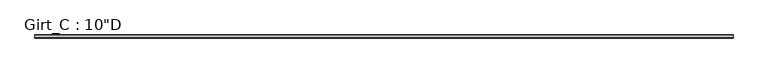
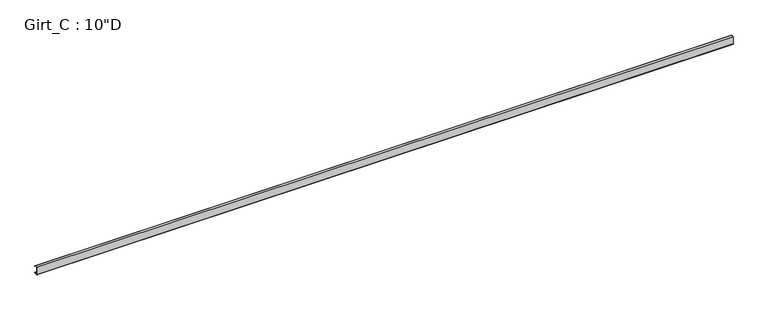
"""IFC4 building model written with IfcOpenShell, lengths in millimetres: beam geometry."""

from ifc_helpers import new_model, si_unit, point, frame, frame_2d, origin, place, context, project, spatial, polyline, circle_curve, trimmed, segment, composite_curve, outline, extrude, source, transform, mapped, element, save


def beam_0e6f5634(model_context):
    return source(origin(), model_context, "Body", "SweptSolid", [
        extrude(outline(composite_curve([segment(polyline([(87.5109375, 127.0), (99.7560415, 112.4068534), (97.6278742, 110.621109), (86.2154765, 124.221875), (3.3005807, 124.221875)]), True, "CONTINUOUS"), segment(trimmed(circle_curve(frame_2d((3.3741066, 122.2381931)), 1.9850441), [point((3.3005807, 124.221875))], [point((1.3890625, 122.2381931))], True, "CARTESIAN"), True, "CONTINUOUS"), segment(polyline([(1.3890625, 122.2381931), (1.3890625, -122.2389339)]), True, "CONTINUOUS"), segment(trimmed(circle_curve(frame_2d((3.3748024, -122.2389339)), 1.9857399), [point((1.3890625, -122.2389339))], [point((3.2694106, -124.221875))], True, "CARTESIAN"), True, "CONTINUOUS"), segment(polyline([(3.2694106, -124.221875), (86.2154765, -124.221875), (97.6510975, -110.5934327), (99.7792647, -112.379177), (87.5109375, -127.0), (3.3734375, -127.0)]), True, "CONTINUOUS"), segment(trimmed(circle_curve(frame_2d((3.3734375, -122.2375)), 4.7625), [point((3.3734375, -127.0))], [point((-1.3890625, -122.2375))], False, "CARTESIAN"), True, "CONTINUOUS"), segment(polyline([(-1.3890625, -122.2375), (-1.3890625, 122.2375)]), True, "CONTINUOUS"), segment(trimmed(circle_curve(frame_2d((3.3734375, 122.2375)), 4.7625), [point((-1.3890625, 122.2375))], [point((3.3734375, 127.0))], False, "CARTESIAN"), True, "CONTINUOUS"), segment(polyline([(3.3734375, 127.0), (87.5109375, 127.0)]), True, "CONTINUOUS")], self_intersect=False)), frame((-11237.4299, 0.0, 0.0), z_axis=(1.0, 0.0, 0.0), x_axis=(0.0, 1.0, 0.0)), (0.0, 0.0, 1.0), 22557.994),
    ])


if __name__ == "__main__":
    model = new_model("IFC4")
    model_context = context("Model", 3, world=origin())
    ifc_project = project(units=[si_unit("LENGTHUNIT", "METRE", prefix="MILLI")], contexts=[model_context])
    site = spatial("IfcSite", under=ifc_project)
    building = spatial("IfcBuilding", under=site)
    placement = place(None, origin())
    beam_shape = beam_0e6f5634(model_context)
    element("IfcBeam", 1, ObjectType="Girt_C : 10\"D", at=placement, inside=building, context=model_context, shape_type="MappedRepresentation", body=[
        mapped(beam_shape, transform((0.0, 0.0, 0.0), x_axis=(1.0, 0.0, 0.0), y_axis=(0.0, 1.0, 0.0), z_axis=(0.0, 0.0, 1.0))),
    ])
    save(model, "model.ifc")

# Revit data of these elements
# Type "Girt_C : 10\"D"
#   half leg = 0' - 1 3/4"
#   Web_Thickness = 0' - 0 7/64"
#   Length [instance default] = 10' - 0"
#   Leg_1 = 0' - 3 1/2"
#   Height = 0' - 10"
#   Structural Material [instance default] = none
